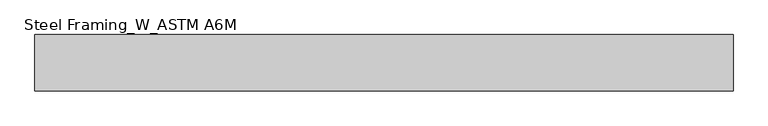
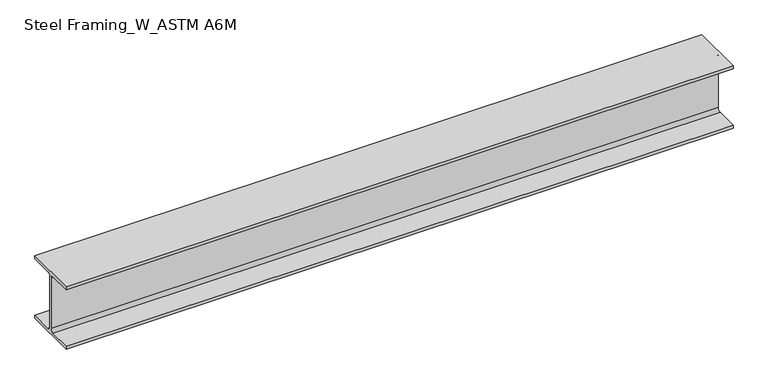
"""IFC4 building model written with IfcOpenShell, lengths in millimetres: beam geometry, Steel Framing_W_ASTM A6M : H_SB_AR_S02_W250x49.1_RCG1."""

from ifc_helpers import new_model, si_unit, point, frame, frame_2d, origin, place, context, project, spatial, polyline, circle_curve, trimmed, segment, composite_curve, outline, extrude, source, transform, mapped, element, save


def steel_framing_w_astm_a6m_1111b065(model_context):
    return source(origin(), model_context, "Body", "SweptSolid", [
        extrude(outline(composite_curve([segment(polyline([(101.0, -112.5), (101.0, -123.5), (-101.0, -123.5), (-101.0, -112.5), (-16.385, -112.5)]), True, "CONTINUOUS"), segment(trimmed(circle_curve(frame_2d((-16.385, -99.8)), 12.7), [point((-16.385, -112.5))], [point((-3.685, -99.8))], True, "CARTESIAN"), True, "CONTINUOUS"), segment(polyline([(-3.685, -99.8), (-3.685, 99.8)]), True, "CONTINUOUS"), segment(trimmed(circle_curve(frame_2d((-16.385, 99.8)), 12.7), [point((-3.685, 99.8))], [point((-16.385, 112.5))], True, "CARTESIAN"), True, "CONTINUOUS"), segment(polyline([(-16.385, 112.5), (-101.0, 112.5), (-101.0, 123.5), (101.0, 123.5), (101.0, 112.5), (16.385, 112.5)]), True, "CONTINUOUS"), segment(trimmed(circle_curve(frame_2d((16.385, 99.8)), 12.7), [point((16.385, 112.5))], [point((3.685, 99.8))], True, "CARTESIAN"), True, "CONTINUOUS"), segment(polyline([(3.685, 99.8), (3.685, -99.8)]), True, "CONTINUOUS"), segment(trimmed(circle_curve(frame_2d((16.385, -99.8)), 12.7), [point((3.685, -99.8))], [point((16.385, -112.5))], True, "CARTESIAN"), True, "CONTINUOUS"), segment(polyline([(16.385, -112.5), (101.0, -112.5)]), True, "CONTINUOUS")], self_intersect=False)), frame((-1243.5, 0.0, 0.0), z_axis=(1.0, 0.0, 0.0), x_axis=(0.0, 1.0, 0.0)), (0.0, 0.0, 1.0), 2499.7),
    ])


if __name__ == "__main__":
    model = new_model("IFC4")
    model_context = context("Model", 3, world=origin())
    ifc_project = project(units=[si_unit("LENGTHUNIT", "METRE", prefix="MILLI")], contexts=[model_context])
    site = spatial("IfcSite", under=ifc_project)
    building = spatial("IfcBuilding", under=site)
    placement = place(None, origin())
    steel_framing_w_astm_a6m_shape = steel_framing_w_astm_a6m_1111b065(model_context)
    element("IfcBeam", 1, ObjectType="Steel Framing_W_ASTM A6M : H_SB_AR_S02_W250x49.1_RCG1", at=placement, inside=building, context=model_context, shape_type="MappedRepresentation", body=[
        mapped(steel_framing_w_astm_a6m_shape, transform((0.0, 0.0, 0.0), x_axis=(1.0, 0.0, 0.0), y_axis=(0.0, 1.0, 0.0), z_axis=(0.0, 0.0, 1.0))),
    ])
    save(model, "model.ifc")

# Revit data of these elements
# Type "Steel Framing_W_ASTM A6M : H_SB_AR_S02_W250x49.1_RCG1"
#   Type Mark = "RCG1"
#   Section Name Key = "W10x33"
#   Width = 20.2 cm
#   Web Thickness = 0.737 cm
#   Web Fillet = 1.27 cm
#   Warping Constant = 212000.0 cm⁶
#   Torsional Moment of Inertia = 24.30 cm⁴
#   Section Area = 62.6 cm²
#   Plastic Modulus weak axis = 229.0 cm³
#   Plastic Modulus strong axis = 636.0 cm³
#   Perimeter = 1.27 m²/m
#   Nominal Weight = 49.10 kgf/m
#   Moment of Inertia weak axis = 1520.00 cm⁴
#   Moment of Inertia strong axis = 7120.00 cm⁴
#   Height = 24.7 cm
#   Flange Thickness = 1.1 cm
#   Elastic Modulus weak axis = 151.0 cm³
#   Elastic Modulus strong axis = 574.0 cm³
#   Centroid Vertical = 12.35 cm
#   Centroid Horizontal = 10.1 cm
#   Length [instance default] = 1500 mm
#   Structural Material [instance default] = Steel, 45-345
#   Bolt Spacing = 0
#   Assembly Code = ""
# Element 1 (IfcBeam, "Steel Framing_W_ASTM A6M : H_SB_AR_S02_W250x49.1_RCG1")
#   Materials on its faces: "Steel, 45-345"
# Materials
#   "Steel, 45-345": class "Metal", colour RGB 189 187 185, transparency 0, Description = "Steel 345 MPa", Cost = 0
